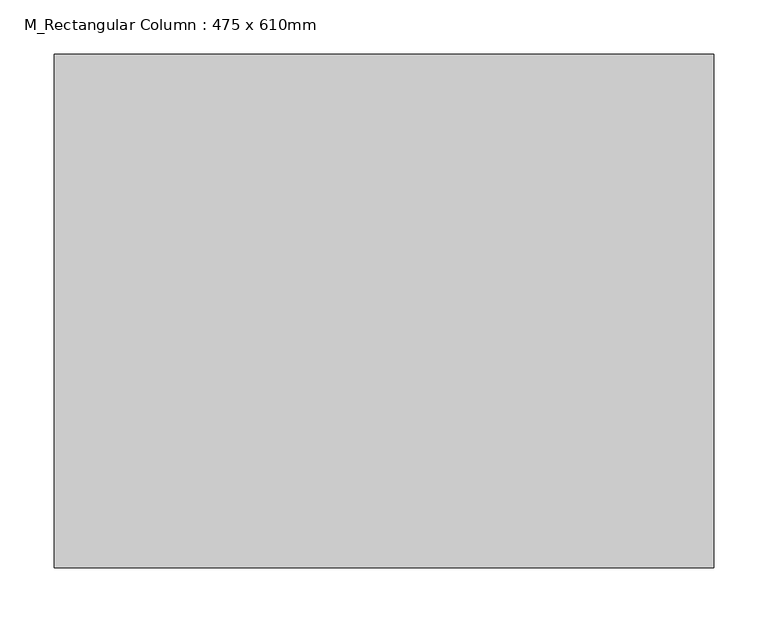
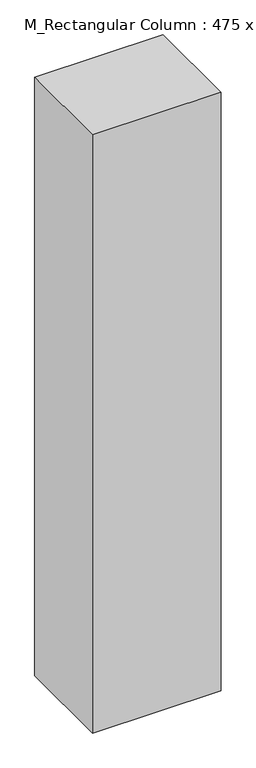
"""IFC4 building model written with IfcOpenShell, lengths in millimetres: column geometry, M_Rectangular Column : 475 x 610mm."""

import ifcopenshell
import ifcopenshell.guid

model = None  # the IFC model being written
_history = None  # IfcOwnerHistory: only IFC2X3 demands one
_inside = {}  # id of a spatial element -> (the spatial element, [elements in it])
_under = {}  # id of a project, library or spatial element -> (it, [spatial elements below it])
_declared = {}  # id of a project -> (the project, [libraries it declares])
_typed = {}  # id of a type object -> (the type object, [elements of that type])
_made_of = {}  # id of a material, layer set ... -> (it, [elements and type objects made of it])


def new_model(schema):
    """Start an empty IFC model of exactly this schema.

    Asked for "IFC4X3", IfcOpenShell would pick the latest addendum, in which some entities
    have other attributes; the version numbers below select the first issue.
    IFC2X3 requires an IfcOwnerHistory on every rooted entity: one is made here for all.
    """
    global model, _history
    if schema == "IFC4X3":
        model = ifcopenshell.file(schema_version=(4, 3, 0, 0))
    else:
        model = ifcopenshell.file(schema=schema)
    _inside.clear()
    _under.clear()
    _declared.clear()
    _typed.clear()
    _made_of.clear()
    _history = None
    if model.schema == "IFC2X3":
        org = make("IfcOrganization", Name="unknown")
        user = make(
            "IfcPersonAndOrganization",
            ThePerson=make("IfcPerson", FamilyName="unknown"),
            TheOrganization=org,
        )
        app = make(
            "IfcApplication",
            ApplicationDeveloper=org,
            Version="unknown",
            ApplicationFullName="unknown",
            ApplicationIdentifier="unknown",
        )
        _history = make(
            "IfcOwnerHistory",
            OwningUser=user,
            OwningApplication=app,
            ChangeAction="ADDED",
            CreationDate=0,
        )
    return model


def make(cls, **values):
    """One entity of the class cls with the attributes given. An attribute that is None is left unset."""
    return model.create_entity(
        cls, **{name: value for name, value in values.items() if value is not None}
    )


def rooted(cls, **values):
    """An entity with a GlobalId (a new one), such as an element, a storey or a relation."""
    return make(cls, GlobalId=ifcopenshell.guid.new(), OwnerHistory=_history, **values)


def si_unit(unit_type, name, prefix=None):
    """IfcSIUnit, for example si_unit("LENGTHUNIT", "METRE", prefix="MILLI")."""
    return make("IfcSIUnit", UnitType=unit_type, Prefix=prefix, Name=name)


def assignment(units):
    """IfcUnitAssignment: the units of a project."""
    return None if units is None else make("IfcUnitAssignment", Units=units)


def point(xyz):
    """IfcCartesianPoint."""
    return None if xyz is None else make("IfcCartesianPoint", Coordinates=xyz)


def direction(xyz):
    """IfcDirection."""
    return None if xyz is None else make("IfcDirection", DirectionRatios=xyz)


def frame(location, z_axis=None, x_axis=None):
    """IfcAxis2Placement3D, a coordinate frame: its origin and axes. An axis left out is left unset."""
    return make(
        "IfcAxis2Placement3D",
        Location=point(location),
        Axis=direction(z_axis),
        RefDirection=direction(x_axis),
    )


def origin():
    """The frame at (0, 0, 0) with its axes left unset."""
    return frame((0.0, 0.0, 0.0))


def origin_with_axes():
    """The frame at (0, 0, 0) with the z axis (0, 0, 1) and the x axis (1, 0, 0) written out."""
    return frame((0.0, 0.0, 0.0), z_axis=(0.0, 0.0, 1.0), x_axis=(1.0, 0.0, 0.0))


def place(relative_to, where):
    """IfcLocalPlacement: puts the frame where relative to a parent placement (None: the world)."""
    return make(
        "IfcLocalPlacement", PlacementRelTo=relative_to, RelativePlacement=where
    )


def context(
    kind, dimensions, precision=None, world=None, true_north=None, identifier=None
):
    """IfcGeometricRepresentationContext, for example the 3D "Model" context."""
    return make(
        "IfcGeometricRepresentationContext",
        ContextIdentifier=identifier,
        ContextType=kind,
        CoordinateSpaceDimension=dimensions,
        Precision=precision,
        WorldCoordinateSystem=world,
        TrueNorth=true_north,
    )


def project(units=None, contexts=None):
    """IfcProject with its units and contexts."""
    return rooted(
        "IfcProject",
        Name="project",
        RepresentationContexts=contexts,
        UnitsInContext=assignment(units),
    )


def spatial(cls, under=None, at=None, **own):
    """A site, building, storey or space (cls), placed at a placement, below another one or the project."""
    s = rooted(cls, ObjectPlacement=at, **own)
    if under is not None:
        _under.setdefault(under.id(), (under, []))[1].append(s)
    return s


def polyline(points):
    """IfcPolyline through the points."""
    return make("IfcPolyline", Points=[point(p) for p in points])


def outline(outer, holes=None, kind="AREA"):
    """IfcArbitraryClosedProfileDef: a profile drawn as a closed curve; with holes, ...WithVoids."""
    if holes is None:
        return make("IfcArbitraryClosedProfileDef", ProfileType=kind, OuterCurve=outer)
    return make(
        "IfcArbitraryProfileDefWithVoids",
        ProfileType=kind,
        OuterCurve=outer,
        InnerCurves=holes,
    )


def extrude(swept, where, along, depth):
    """IfcExtrudedAreaSolid: the profile swept, set in the frame where, extruded along a direction by depth."""
    return make(
        "IfcExtrudedAreaSolid",
        SweptArea=swept,
        Position=where,
        ExtrudedDirection=direction(along),
        Depth=depth,
    )


def shape(context_of_items, identifier, shape_type, items):
    """IfcShapeRepresentation: the items that make up one representation, for example the "Body"."""
    return make(
        "IfcShapeRepresentation",
        ContextOfItems=context_of_items,
        RepresentationIdentifier=identifier,
        RepresentationType=shape_type,
        Items=items,
    )


def source(mapping_origin, context_of_items, identifier, shape_type, items):
    """IfcRepresentationMap: a shape defined once, which mapped items show again and again."""
    return make(
        "IfcRepresentationMap",
        MappingOrigin=mapping_origin,
        MappedRepresentation=shape(context_of_items, identifier, shape_type, items),
    )


def transform(
    local_origin,
    x_axis=None,
    y_axis=None,
    z_axis=None,
    scale=None,
    scale2=None,
    scale3=None,
    uniform=True,
):
    """IfcCartesianTransformationOperator3D, or its non-uniform kind. x_axis, y_axis, z_axis: its Axis1, 2, 3."""
    if uniform:
        return make(
            "IfcCartesianTransformationOperator3D",
            Axis1=direction(x_axis),
            Axis2=direction(y_axis),
            LocalOrigin=point(local_origin),
            Scale=scale,
            Axis3=direction(z_axis),
        )
    return make(
        "IfcCartesianTransformationOperator3DnonUniform",
        Axis1=direction(x_axis),
        Axis2=direction(y_axis),
        LocalOrigin=point(local_origin),
        Scale=scale,
        Axis3=direction(z_axis),
        Scale2=scale2,
        Scale3=scale3,
    )


def mapped(mapping_source, mapping_target):
    """IfcMappedItem: shows the shape of a source again, moved by a transform."""
    return make(
        "IfcMappedItem", MappingSource=mapping_source, MappingTarget=mapping_target
    )


def made_of(thing, what):
    """Note that an element or type object is made of a material, layer set ...; save() writes the relation."""
    if what is not None:
        _made_of.setdefault(what.id(), (what, []))[1].append(thing)
    return thing


def element(
    cls,
    number,
    at=None,
    inside=None,
    cuts=None,
    type_object=None,
    material=None,
    context=None,
    identifier="Body",
    shape_type=None,
    held_by="IfcProductDefinitionShape",
    body=None,
    shapes=None,
    **own,
):
    """One element of the class cls, such as IfcWall. Its Tag is "e" and its number.

    at: its placement. inside: the storey or other place that contains it. cuts: it is an
    opening in that element (IfcRelVoidsElement). A single representation is given by context,
    identifier, shape_type and body (its items); several are given by shapes. held_by: the class
    of the entity that holds the representations. save() writes the other relations.
    """
    e = rooted(cls, Tag="e%d" % number, ObjectPlacement=at, **own)
    if body is not None:
        shapes = [shape(context, identifier, shape_type, body)]
    if shapes is not None:
        e.Representation = make(held_by, Representations=shapes)
    if inside is not None:
        _inside.setdefault(inside.id(), (inside, []))[1].append(e)
    if cuts is not None:
        rooted(
            "IfcRelVoidsElement", RelatingBuildingElement=cuts, RelatedOpeningElement=e
        )
    if type_object is not None:
        _typed.setdefault(type_object.id(), (type_object, []))[1].append(e)
    return made_of(e, material)


def aggregate(whole, parts):
    """IfcRelAggregates: a whole, such as a stair, and the parts it consists of."""
    return rooted("IfcRelAggregates", RelatingObject=whole, RelatedObjects=parts)


def save(model, path):
    """Write the relations noted so far, then the file.

    IfcRelAggregates (storeys below a building ...), IfcRelContainedInSpatialStructure (elements
    in a storey), IfcRelDefinesByType, IfcRelAssociatesMaterial and IfcRelDeclares: one each for
    every whole, place, type object, material and project.
    """
    for whole, parts in _under.values():
        aggregate(whole, parts)
    for where, things in _inside.values():
        rooted(
            "IfcRelContainedInSpatialStructure",
            RelatedElements=things,
            RelatingStructure=where,
        )
    for kind, things in _typed.values():
        rooted("IfcRelDefinesByType", RelatedObjects=things, RelatingType=kind)
    for what, things in _made_of.values():
        rooted("IfcRelAssociatesMaterial", RelatedObjects=things, RelatingMaterial=what)
    for by, libraries in _declared.values():
        rooted("IfcRelDeclares", RelatingContext=by, RelatedDefinitions=libraries)
    model.write(path)


def m_rectangular_column_475_x_610mm_f11b4c06(model_context):
    return source(origin(), model_context, "Body", "SweptSolid", [
        extrude(outline(polyline([(305.0, 237.5), (305.0, -237.5), (-305.0, -237.5), (-305.0, 237.5), (305.0, 237.5)])), origin_with_axes(), (0.0, 0.0, 1.0), 3000.0),
    ])


if __name__ == "__main__":
    model = new_model("IFC4")
    model_context = context("Model", 3, world=origin())
    ifc_project = project(units=[si_unit("LENGTHUNIT", "METRE", prefix="MILLI")], contexts=[model_context])
    site = spatial("IfcSite", under=ifc_project)
    building = spatial("IfcBuilding", under=site)
    placement = place(None, origin())
    m_rectangular_column_475_x_610mm_shape = m_rectangular_column_475_x_610mm_f11b4c06(model_context)
    element("IfcColumn", 1, ObjectType="M_Rectangular Column : 475 x 610mm", at=placement, inside=building, context=model_context, shape_type="MappedRepresentation", body=[
        mapped(m_rectangular_column_475_x_610mm_shape, transform((0.0, 0.0, 0.0), x_axis=(1.0, 0.0, 0.0), y_axis=(0.0, 1.0, 0.0), z_axis=(0.0, 0.0, 1.0))),
    ])
    save(model, "model.ifc")

# Revit data of these elements
# Type "M_Rectangular Column : 475 x 610mm"
#   Depth = 475 mm
#   Offset Base = 0 mm
#   Offset Top = 0 mm
#   Width = 610 mm
#   Material = none
